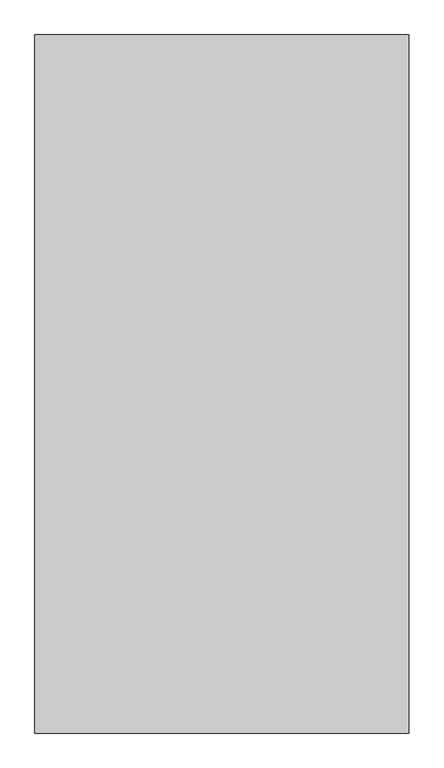
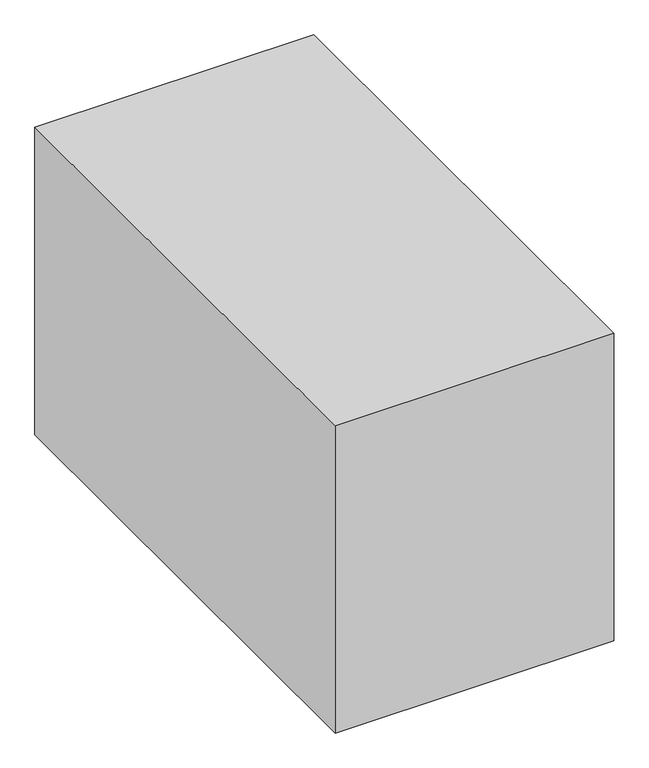
"""IFC4 building model written with IfcOpenShell, lengths in millimetres: proxy geometry, Space Planning Box_hec : Space Planning Box_hec."""

from ifc_helpers import new_model, si_unit, origin, origin_with_axes, place, context, project, spatial, polyline, outline, extrude, source, transform, mapped, element, save


def generic_models_f42d0df8(model_context):
    return source(origin(), model_context, "Body", "SweptSolid", [
        extrude(outline(polyline([(1500.0, 2800.0), (1500.0, -2800.0), (-1500.0, -2800.0), (-1500.0, 2800.0), (1500.0, 2800.0)])), origin_with_axes(), (0.0, 0.0, 1.0), 3500.0),
    ])


if __name__ == "__main__":
    model = new_model("IFC4")
    model_context = context("Model", 3, world=origin())
    ifc_project = project(units=[si_unit("LENGTHUNIT", "METRE", prefix="MILLI")], contexts=[model_context])
    site = spatial("IfcSite", under=ifc_project)
    building = spatial("IfcBuilding", under=site)
    placement = place(None, origin())
    generic_models_shape = generic_models_f42d0df8(model_context)
    element("IfcBuildingElementProxy", 1, Name="Space Planning Box_hec : Space Planning Box_hec", ObjectType="Space Planning Box_hec : Space Planning Box_hec", at=placement, inside=building, context=model_context, shape_type="MappedRepresentation", body=[
        mapped(generic_models_shape, transform((0.0, 0.0, 0.0), x_axis=(1.0, 0.0, 0.0), y_axis=(0.0, 1.0, 0.0), z_axis=(0.0, 0.0, 1.0))),
    ])
    save(model, "model.ifc")

# Revit data of these elements
# Type "Space Planning Box_hec : Space Planning Box_hec"
#   Type Comments = "..."
#   Room Name [instance default] = "?"
#   Interior Finish [instance default] = ""
#   Exterior Finish [instance default] = ""
#   Department [instance default] = ""
#   Assembly Code = "..."
#   ceiling height [instance default] = 0
#   Width [instance default] = 1524 mm
#   Program Area [instance default] = 0.00 m²
#   Length [instance default] = 1524 mm
#   Height [instance default] = 1524 mm
#   Area [instance default] = 2.32258 m²
#   Fill Color [instance default] = Cyan
#   Default Elevation = 0
# Element 1 (IfcBuildingElementProxy, "Space Planning Box_hec : Space Planning Box_hec")
#   Room Name = "Toilet(F)"
#   Exterior Finish = "RF1..N/A,,N/A..N/A..N/A"
#   Department = "AR"
#   Width = 3000 mm
#   Program Area = 16.80 m²
#   Length = 5600 mm
#   Height = 3500 mm
#   Area = 16.80 m²
#   Materials on its faces: "Cyan"
# Materials
#   "Cyan": class "Generic", colour RGB 0 255 255, transparency 0.2, Cost = 0
